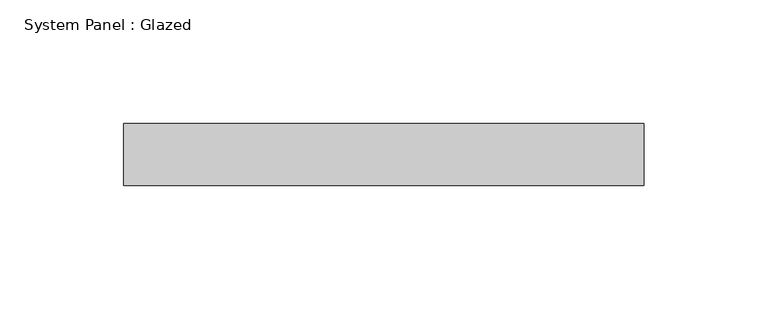
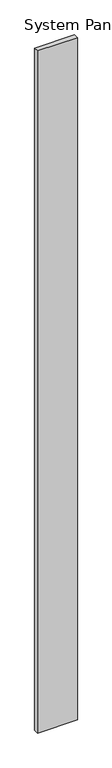
"""IFC4 building model written with IfcOpenShell, lengths in millimetres: plate geometry, System Panel : Glazed."""

from ifc_helpers import new_model, si_unit, origin, origin_with_axes, place, context, project, spatial, polyline, outline, extrude, source, transform, mapped, element, save


def system_panel_glazed_31375f6b(model_context):
    return source(origin(), model_context, "Body", "SweptSolid", [
        extrude(outline(polyline([(104.9999998, 24.5), (-104.9999998, 24.5), (-104.9999998, 49.5), (104.9999998, 49.5), (104.9999998, 24.5)])), origin_with_axes(), (0.0, 0.0, 1.0), 3800.0),
    ])


if __name__ == "__main__":
    model = new_model("IFC4")
    model_context = context("Model", 3, world=origin())
    ifc_project = project(units=[si_unit("LENGTHUNIT", "METRE", prefix="MILLI")], contexts=[model_context])
    site = spatial("IfcSite", under=ifc_project)
    building = spatial("IfcBuilding", under=site)
    placement = place(None, origin())
    system_panel_glazed_shape = system_panel_glazed_31375f6b(model_context)
    element("IfcPlate", 1, ObjectType="System Panel : Glazed", at=placement, inside=building, context=model_context, shape_type="MappedRepresentation", body=[
        mapped(system_panel_glazed_shape, transform((0.0, 0.0, 0.0), x_axis=(1.0, 0.0, 0.0), y_axis=(0.0, 1.0, 0.0), z_axis=(0.0, 0.0, 1.0))),
    ])
    save(model, "model.ifc")

# Revit data of these elements
# Type "System Panel : Glazed"
#   Construction Type Id = "GSP4R"
#   Analytic Construction = "1/8 in Pilkington single glazing"
#   Visual Light Transmittance = 0.9
#   Solar Heat Gain Coefficient = 0.86
#   Heat Transfer Coefficient (U) = 6.7069 W/(m²·K)
#   Define Thermal Properties by = 1
# Element 1 (IfcPlate, "System Panel : Glazed")
#   Materials on its faces: "Glass"
# Materials
#   "Glass": class "Glass", colour RGB 0 128 192, transparency 0.9, Description = "Soda Lime Glass", Cost = 0
